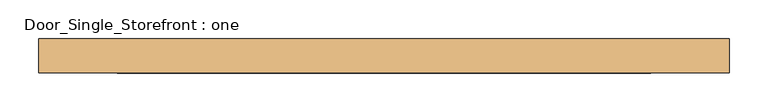
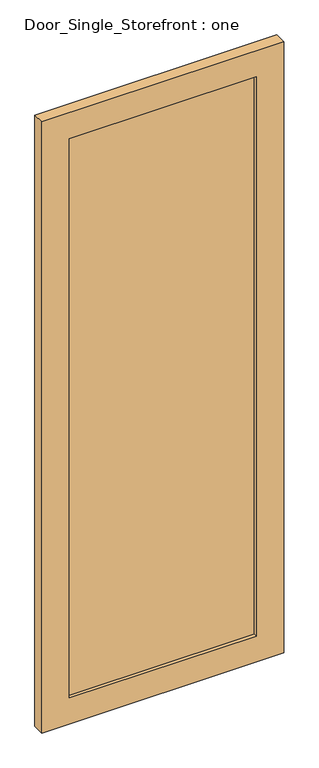
"""IFC4 building model written with IfcOpenShell, lengths in millimetres: door geometry, Door_Single_Storefront : one."""

from ifc_helpers import new_model, si_unit, frame, origin, place, context, project, spatial, polyline, outline, extrude, source, transform, mapped, element, save


def door_single_storefront_one_901062f1(model_context):
    return source(origin(), model_context, "Body", "SweptSolid", [
        extrude(outline(polyline([(2387.6, -446.88125), (0.0, -446.88125), (0.0, 446.88125), (2387.6, 446.88125), (2387.6, -446.88125)]), holes=[polyline([(101.6, 345.28125), (101.6, -345.28125), (2286.0, -345.28125), (2286.0, 345.28125), (101.6, 345.28125)])]), frame((0.0, 6.35, 0.0), z_axis=(0.0, 1.0, 0.0), x_axis=(0.0, 0.0, 1.0)), (0.0, 0.0, 1.0), 44.45),
        extrude(outline(polyline([(345.28125, 19.05), (-345.28125, 19.05), (-345.28125, 38.1), (345.28125, 38.1), (345.28125, 19.05)])), frame((0.0, 0.0, 101.6), z_axis=(0.0, 0.0, 1.0), x_axis=(1.0, 0.0, 0.0)), (0.0, 0.0, 1.0), 2184.4),
    ])


if __name__ == "__main__":
    model = new_model("IFC4")
    model_context = context("Model", 3, world=origin())
    ifc_project = project(units=[si_unit("LENGTHUNIT", "METRE", prefix="MILLI")], contexts=[model_context])
    site = spatial("IfcSite", under=ifc_project)
    building = spatial("IfcBuilding", under=site)
    placement = place(None, origin())
    door_single_storefront_one_shape = door_single_storefront_one_901062f1(model_context)
    element("IfcDoor", 1, ObjectType="Door_Single_Storefront : one", at=placement, inside=building, context=model_context, shape_type="MappedRepresentation", body=[
        mapped(door_single_storefront_one_shape, transform((0.0, 0.0, 0.0), x_axis=(1.0, 0.0, 0.0), y_axis=(0.0, 1.0, 0.0), z_axis=(0.0, 0.0, 1.0))),
    ])
    save(model, "model.ifc")

# Revit data of these elements
# Type "Door_Single_Storefront : one"
#   Type Mark = "27"
#   Analytic Construction = "<None>"
#   Stile_Width = 0' - 4"
#   Door_Thickness = 0' - 1 3/4"
#   Door_Offset = 0' - 2"
#   Glass_Material = Glass
#   Frame_Material = Aluminum
#   Function = (empty or 0)
# Element 1 (IfcDoor, "Door_Single_Storefront : one")
#   Materials on its faces: "Aluminum", "Glass"
# Materials
#   "Glass": class "Glass", colour RGB 0 128 192, transparency 0.75, Description = "Soda Lime Glass", Cost = 0
#   "Aluminum": class "Metal", colour RGB 247 247 247, transparency 0, Description = "Aluminum 6061", Cost = 0
